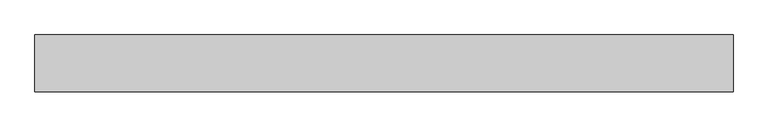
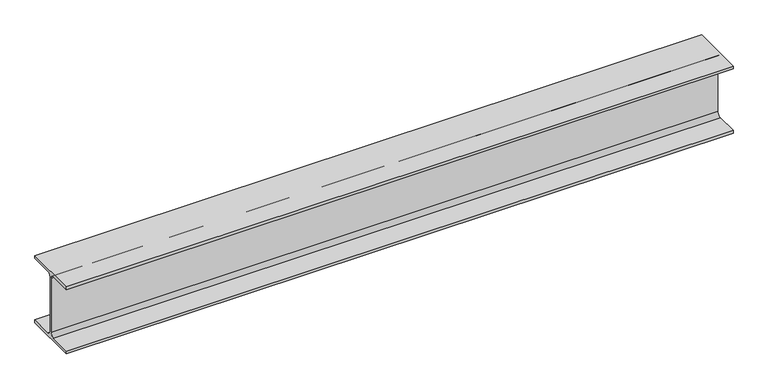
"""IFC4 building model written with IfcOpenShell, lengths in millimetres: beam geometry, 0912_Steel Framing_H-KSD3502 : H_SB_ASB_H-390x300x10x16."""

import ifcopenshell
import ifcopenshell.guid

model = None  # the IFC model being written
_history = None  # IfcOwnerHistory: only IFC2X3 demands one
_inside = {}  # id of a spatial element -> (the spatial element, [elements in it])
_under = {}  # id of a project, library or spatial element -> (it, [spatial elements below it])
_declared = {}  # id of a project -> (the project, [libraries it declares])
_typed = {}  # id of a type object -> (the type object, [elements of that type])
_made_of = {}  # id of a material, layer set ... -> (it, [elements and type objects made of it])


def new_model(schema):
    """Start an empty IFC model of exactly this schema.

    Asked for "IFC4X3", IfcOpenShell would pick the latest addendum, in which some entities
    have other attributes; the version numbers below select the first issue.
    IFC2X3 requires an IfcOwnerHistory on every rooted entity: one is made here for all.
    """
    global model, _history
    if schema == "IFC4X3":
        model = ifcopenshell.file(schema_version=(4, 3, 0, 0))
    else:
        model = ifcopenshell.file(schema=schema)
    _inside.clear()
    _under.clear()
    _declared.clear()
    _typed.clear()
    _made_of.clear()
    _history = None
    if model.schema == "IFC2X3":
        org = make("IfcOrganization", Name="unknown")
        user = make(
            "IfcPersonAndOrganization",
            ThePerson=make("IfcPerson", FamilyName="unknown"),
            TheOrganization=org,
        )
        app = make(
            "IfcApplication",
            ApplicationDeveloper=org,
            Version="unknown",
            ApplicationFullName="unknown",
            ApplicationIdentifier="unknown",
        )
        _history = make(
            "IfcOwnerHistory",
            OwningUser=user,
            OwningApplication=app,
            ChangeAction="ADDED",
            CreationDate=0,
        )
    return model


def make(cls, **values):
    """One entity of the class cls with the attributes given. An attribute that is None is left unset."""
    return model.create_entity(
        cls, **{name: value for name, value in values.items() if value is not None}
    )


def rooted(cls, **values):
    """An entity with a GlobalId (a new one), such as an element, a storey or a relation."""
    return make(cls, GlobalId=ifcopenshell.guid.new(), OwnerHistory=_history, **values)


def si_unit(unit_type, name, prefix=None):
    """IfcSIUnit, for example si_unit("LENGTHUNIT", "METRE", prefix="MILLI")."""
    return make("IfcSIUnit", UnitType=unit_type, Prefix=prefix, Name=name)


def assignment(units):
    """IfcUnitAssignment: the units of a project."""
    return None if units is None else make("IfcUnitAssignment", Units=units)


def point(xyz):
    """IfcCartesianPoint."""
    return None if xyz is None else make("IfcCartesianPoint", Coordinates=xyz)


def direction(xyz):
    """IfcDirection."""
    return None if xyz is None else make("IfcDirection", DirectionRatios=xyz)


def frame(location, z_axis=None, x_axis=None):
    """IfcAxis2Placement3D, a coordinate frame: its origin and axes. An axis left out is left unset."""
    return make(
        "IfcAxis2Placement3D",
        Location=point(location),
        Axis=direction(z_axis),
        RefDirection=direction(x_axis),
    )


def frame_2d(location, x_axis=None):
    """IfcAxis2Placement2D, a coordinate frame in the plane: its origin and x axis."""
    return make(
        "IfcAxis2Placement2D", Location=point(location), RefDirection=direction(x_axis)
    )


def origin():
    """The frame at (0, 0, 0) with its axes left unset."""
    return frame((0.0, 0.0, 0.0))


def place(relative_to, where):
    """IfcLocalPlacement: puts the frame where relative to a parent placement (None: the world)."""
    return make(
        "IfcLocalPlacement", PlacementRelTo=relative_to, RelativePlacement=where
    )


def context(
    kind, dimensions, precision=None, world=None, true_north=None, identifier=None
):
    """IfcGeometricRepresentationContext, for example the 3D "Model" context."""
    return make(
        "IfcGeometricRepresentationContext",
        ContextIdentifier=identifier,
        ContextType=kind,
        CoordinateSpaceDimension=dimensions,
        Precision=precision,
        WorldCoordinateSystem=world,
        TrueNorth=true_north,
    )


def project(units=None, contexts=None):
    """IfcProject with its units and contexts."""
    return rooted(
        "IfcProject",
        Name="project",
        RepresentationContexts=contexts,
        UnitsInContext=assignment(units),
    )


def spatial(cls, under=None, at=None, **own):
    """A site, building, storey or space (cls), placed at a placement, below another one or the project."""
    s = rooted(cls, ObjectPlacement=at, **own)
    if under is not None:
        _under.setdefault(under.id(), (under, []))[1].append(s)
    return s


def polyline(points):
    """IfcPolyline through the points."""
    return make("IfcPolyline", Points=[point(p) for p in points])


def circle_curve(where, radius):
    """IfcCircle in the frame where."""
    return make("IfcCircle", Position=where, Radius=radius)


def trimmed(basis, trim1, trim2, sense, master):
    """IfcTrimmedCurve: the piece of a basis curve between two trims."""
    return make(
        "IfcTrimmedCurve",
        BasisCurve=basis,
        Trim1=trim1,
        Trim2=trim2,
        SenseAgreement=sense,
        MasterRepresentation=master,
    )


def segment(curve, same_sense, transition):
    """IfcCompositeCurveSegment."""
    return make(
        "IfcCompositeCurveSegment",
        Transition=transition,
        SameSense=same_sense,
        ParentCurve=curve,
    )


def composite_curve(segments, self_intersect=None):
    """IfcCompositeCurve: segments joined end to end."""
    return make("IfcCompositeCurve", Segments=segments, SelfIntersect=self_intersect)


def outline(outer, holes=None, kind="AREA"):
    """IfcArbitraryClosedProfileDef: a profile drawn as a closed curve; with holes, ...WithVoids."""
    if holes is None:
        return make("IfcArbitraryClosedProfileDef", ProfileType=kind, OuterCurve=outer)
    return make(
        "IfcArbitraryProfileDefWithVoids",
        ProfileType=kind,
        OuterCurve=outer,
        InnerCurves=holes,
    )


def extrude(swept, where, along, depth):
    """IfcExtrudedAreaSolid: the profile swept, set in the frame where, extruded along a direction by depth."""
    return make(
        "IfcExtrudedAreaSolid",
        SweptArea=swept,
        Position=where,
        ExtrudedDirection=direction(along),
        Depth=depth,
    )


def shape(context_of_items, identifier, shape_type, items):
    """IfcShapeRepresentation: the items that make up one representation, for example the "Body"."""
    return make(
        "IfcShapeRepresentation",
        ContextOfItems=context_of_items,
        RepresentationIdentifier=identifier,
        RepresentationType=shape_type,
        Items=items,
    )


def source(mapping_origin, context_of_items, identifier, shape_type, items):
    """IfcRepresentationMap: a shape defined once, which mapped items show again and again."""
    return make(
        "IfcRepresentationMap",
        MappingOrigin=mapping_origin,
        MappedRepresentation=shape(context_of_items, identifier, shape_type, items),
    )


def transform(
    local_origin,
    x_axis=None,
    y_axis=None,
    z_axis=None,
    scale=None,
    scale2=None,
    scale3=None,
    uniform=True,
):
    """IfcCartesianTransformationOperator3D, or its non-uniform kind. x_axis, y_axis, z_axis: its Axis1, 2, 3."""
    if uniform:
        return make(
            "IfcCartesianTransformationOperator3D",
            Axis1=direction(x_axis),
            Axis2=direction(y_axis),
            LocalOrigin=point(local_origin),
            Scale=scale,
            Axis3=direction(z_axis),
        )
    return make(
        "IfcCartesianTransformationOperator3DnonUniform",
        Axis1=direction(x_axis),
        Axis2=direction(y_axis),
        LocalOrigin=point(local_origin),
        Scale=scale,
        Axis3=direction(z_axis),
        Scale2=scale2,
        Scale3=scale3,
    )


def mapped(mapping_source, mapping_target):
    """IfcMappedItem: shows the shape of a source again, moved by a transform."""
    return make(
        "IfcMappedItem", MappingSource=mapping_source, MappingTarget=mapping_target
    )


def made_of(thing, what):
    """Note that an element or type object is made of a material, layer set ...; save() writes the relation."""
    if what is not None:
        _made_of.setdefault(what.id(), (what, []))[1].append(thing)
    return thing


def element(
    cls,
    number,
    at=None,
    inside=None,
    cuts=None,
    type_object=None,
    material=None,
    context=None,
    identifier="Body",
    shape_type=None,
    held_by="IfcProductDefinitionShape",
    body=None,
    shapes=None,
    **own,
):
    """One element of the class cls, such as IfcWall. Its Tag is "e" and its number.

    at: its placement. inside: the storey or other place that contains it. cuts: it is an
    opening in that element (IfcRelVoidsElement). A single representation is given by context,
    identifier, shape_type and body (its items); several are given by shapes. held_by: the class
    of the entity that holds the representations. save() writes the other relations.
    """
    e = rooted(cls, Tag="e%d" % number, ObjectPlacement=at, **own)
    if body is not None:
        shapes = [shape(context, identifier, shape_type, body)]
    if shapes is not None:
        e.Representation = make(held_by, Representations=shapes)
    if inside is not None:
        _inside.setdefault(inside.id(), (inside, []))[1].append(e)
    if cuts is not None:
        rooted(
            "IfcRelVoidsElement", RelatingBuildingElement=cuts, RelatedOpeningElement=e
        )
    if type_object is not None:
        _typed.setdefault(type_object.id(), (type_object, []))[1].append(e)
    return made_of(e, material)


def aggregate(whole, parts):
    """IfcRelAggregates: a whole, such as a stair, and the parts it consists of."""
    return rooted("IfcRelAggregates", RelatingObject=whole, RelatedObjects=parts)


def save(model, path):
    """Write the relations noted so far, then the file.

    IfcRelAggregates (storeys below a building ...), IfcRelContainedInSpatialStructure (elements
    in a storey), IfcRelDefinesByType, IfcRelAssociatesMaterial and IfcRelDeclares: one each for
    every whole, place, type object, material and project.
    """
    for whole, parts in _under.values():
        aggregate(whole, parts)
    for where, things in _inside.values():
        rooted(
            "IfcRelContainedInSpatialStructure",
            RelatedElements=things,
            RelatingStructure=where,
        )
    for kind, things in _typed.values():
        rooted("IfcRelDefinesByType", RelatedObjects=things, RelatingType=kind)
    for what, things in _made_of.values():
        rooted("IfcRelAssociatesMaterial", RelatedObjects=things, RelatingMaterial=what)
    for by, libraries in _declared.values():
        rooted("IfcRelDeclares", RelatingContext=by, RelatedDefinitions=libraries)
    model.write(path)


def beam_7f1fef08(model_context):
    return source(origin(), model_context, "Body", "SweptSolid", [
        extrude(outline(composite_curve([segment(polyline([(150.0, -179.0), (150.0, -195.0), (-150.0, -195.0), (-150.0, -179.0), (-27.0, -179.0)]), True, "CONTINUOUS"), segment(trimmed(circle_curve(frame_2d((-27.0, -157.0)), 22.0), [point((-27.0, -179.0))], [point((-5.0, -157.0))], True, "CARTESIAN"), True, "CONTINUOUS"), segment(polyline([(-5.0, -157.0), (-5.0, 157.0)]), True, "CONTINUOUS"), segment(trimmed(circle_curve(frame_2d((-27.0, 157.0)), 22.0), [point((-5.0, 157.0))], [point((-27.0, 179.0))], True, "CARTESIAN"), True, "CONTINUOUS"), segment(polyline([(-27.0, 179.0), (-150.0, 179.0), (-150.0, 195.0), (150.0, 195.0), (150.0, 179.0), (27.0, 179.0)]), True, "CONTINUOUS"), segment(trimmed(circle_curve(frame_2d((27.0, 157.0)), 22.0), [point((27.0, 179.0))], [point((5.0, 157.0))], True, "CARTESIAN"), True, "CONTINUOUS"), segment(polyline([(5.0, 157.0), (5.0, -157.0)]), True, "CONTINUOUS"), segment(trimmed(circle_curve(frame_2d((27.0, -157.0)), 22.0), [point((5.0, -157.0))], [point((27.0, -179.0))], True, "CARTESIAN"), True, "CONTINUOUS"), segment(polyline([(27.0, -179.0), (150.0, -179.0)]), True, "CONTINUOUS")], self_intersect=False)), frame((-1837.3, 0.0, 0.0), z_axis=(1.0, 0.0, 0.0), x_axis=(0.0, 1.0, 0.0)), (0.0, 0.0, 1.0), 3674.6),
    ])


if __name__ == "__main__":
    model = new_model("IFC4")
    model_context = context("Model", 3, world=origin())
    ifc_project = project(units=[si_unit("LENGTHUNIT", "METRE", prefix="MILLI")], contexts=[model_context])
    site = spatial("IfcSite", under=ifc_project)
    building = spatial("IfcBuilding", under=site)
    placement = place(None, origin())
    beam_shape = beam_7f1fef08(model_context)
    element("IfcBeam", 1, ObjectType="0912_Steel Framing_H-KSD3502 : H_SB_ASB_H-390x300x10x16", at=placement, inside=building, context=model_context, shape_type="MappedRepresentation", body=[
        mapped(beam_shape, transform((0.0, 0.0, 0.0), x_axis=(1.0, 0.0, 0.0), y_axis=(0.0, 1.0, 0.0), z_axis=(0.0, 0.0, 1.0))),
    ])
    save(model, "model.ifc")

# Revit data of these elements
# Type "0912_Steel Framing_H-KSD3502 : H_SB_ASB_H-390x300x10x16"
#   H_WM Code_1 = "S01AA001-00001 | Main Steel Structure Fabrication Work | Shelter/Building | Heavy Steel - Standard (Weight≥90KG/M) | Material: (   )"
#   H_WM Code_2 = "S03AA027-00001 | Main Steel Structure Erection Work | Shelter/Building | Heavy Steel (Weight≥90KG/M) | Material: (   )"
#   H_WM Code_3 = "S01AA010-00001 | Main Steel Structure Fabrication Work | Shelter/Building | Steel Painting/Coating | for Non-Fireproofed Steel Surface, Surface Preparation, Primer, Second & Final Coat | Material: (   )"
#   H_Q'ty Cal Type Tag = "SB-Q2"
#   Width = 30.0 cm
#   Web Thickness = 1.0 cm
#   Web Fillet = 2.2 cm
#   Warping Constant = 2520000.0 cm⁶
#   W = 0
#   Torsional Moment of Inertia = 94.3867 cm⁴
#   Section Area = 136.0 cm²
#   Plastic Modulus weak axis = 733.0 cm³
#   Plastic Modulus strong axis = 2190.0 cm³
#   Perimeter = 1.92 m²/m
#   Nominal Weight = 107.00 kgf/m
#   Moment of Inertia weak axis = 7210.00 cm⁴
#   Moment of Inertia strong axis = 38700.00 cm⁴
#   Height = 39.0 cm
#   Flange Thickness = 1.6 cm
#   Elastic Modulus weak axis = 481.0 cm³
#   Elastic Modulus strong axis = 1980.0 cm³
#   Centroid Vertical = 19.5 cm
#   Centroid Horizontal = 15.0 cm
#   Ix = 387000000
#   Length [instance default] = 1.5240 m
#   Zx = 2190000
#   b = 0.3000 m
#   h = 0.3900 m
#   r = 0.0220 m
#   s = 0.0100 m
#   t = 0.0160 m
#   A = 0.0136 m²
#   Structural Material [instance default] = Steel, 45-345
#   Assembly Code = ""
# Element 1 (IfcBeam, "0912_Steel Framing_H-KSD3502 : H_SB_ASB_H-390x300x10x16")
#   Structural Material = none
# Materials
#   "Steel, 45-345": class "Metal", colour RGB 189 187 185, transparency 0, Description = "Steel 345 MPa", Cost = 0
